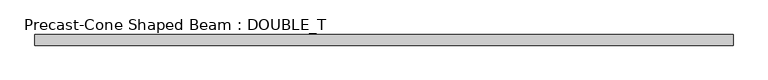
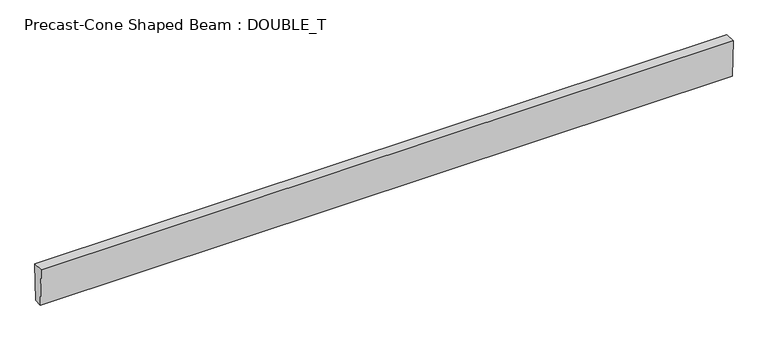
"""IFC4 building model written with IfcOpenShell, lengths in millimetres: beam geometry, Precast-Cone Shaped Beam : DOUBLE_T."""

from ifc_helpers import new_model, si_unit, frame, origin, place, context, project, spatial, polyline, outline, extrude, source, transform, mapped, element, save


def precast_cone_shaped_beam_double_t_e3fa137c(model_context):
    return source(origin(), model_context, "Body", "SweptSolid", [
        extrude(outline(polyline([(50.8, -228.6), (-50.8, -228.6), (-63.5, 228.6), (63.5, 228.6), (50.8, -228.6)])), frame((-4296.56875, 0.0, 0.0), z_axis=(1.0, 0.0, 0.0), x_axis=(0.0, 1.0, 0.0)), (0.0, 0.0, 1.0), 8318.5),
    ])


if __name__ == "__main__":
    model = new_model("IFC4")
    model_context = context("Model", 3, world=origin())
    ifc_project = project(units=[si_unit("LENGTHUNIT", "METRE", prefix="MILLI")], contexts=[model_context])
    site = spatial("IfcSite", under=ifc_project)
    building = spatial("IfcBuilding", under=site)
    placement = place(None, origin())
    precast_cone_shaped_beam_double_t_shape = precast_cone_shaped_beam_double_t_e3fa137c(model_context)
    element("IfcBeam", 1, ObjectType="Precast-Cone Shaped Beam : DOUBLE_T", at=placement, inside=building, context=model_context, shape_type="MappedRepresentation", body=[
        mapped(precast_cone_shaped_beam_double_t_shape, transform((0.0, 0.0, 0.0), x_axis=(1.0, 0.0, 0.0), y_axis=(0.0, 1.0, 0.0), z_axis=(0.0, 0.0, 1.0))),
    ])
    save(model, "model.ifc")

# Revit data of these elements
# Type "Precast-Cone Shaped Beam : DOUBLE_T"
#   Top Width = 0' - 5"
#   Tie Rod Weight [instance default] = 30
#   Tie Rod W [instance default] = 0.0660938 kip
#   Single Rebar Weight [instance default] = 50
#   Single Rebar W [instance default] = 0.110156 kip
#   Rebar Grids Weight [instance default] = 100
#   Rebar Grids W [instance default] = 0.220313 kip
#   Depth = 1' - 6"
#   Bottom Width = 0' - 4"
#   Length [instance default] = 5' - 0"
#   Structural Material [instance default] = Concrete, Precast
#   Assembly Code = ""
# Element 1 (IfcBeam, "Precast-Cone Shaped Beam : DOUBLE_T")
#   Length = 27' - 5 11/16"
#   Structural Material = Concrete - Precast Concrete - Normal Weight Concrete - 5 ksi
#   Materials on its faces: "Concrete - Precast Concrete - Normal Weight Concrete - 5 ksi"
# Materials
#   "Concrete, Precast": class "Concrete", colour RGB 198 187 187, transparency 0, Description = "Precast concrete", Cost = 0
#   "Concrete - Precast Concrete - Normal Weight Concrete - 5 ksi": class "Concrete", colour RGB 198 187 187, transparency 0, Cost = 0
